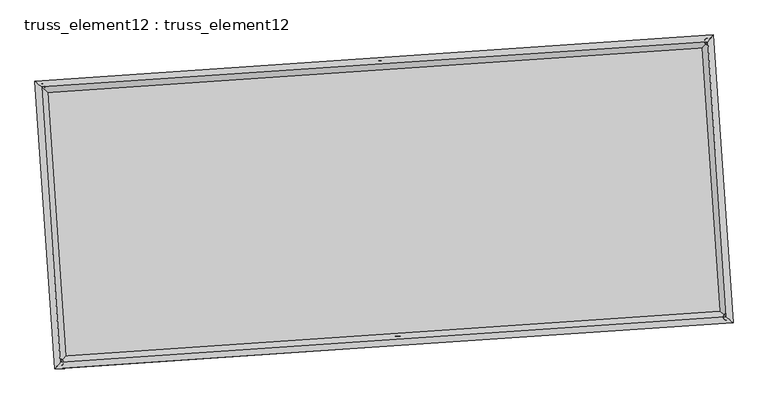
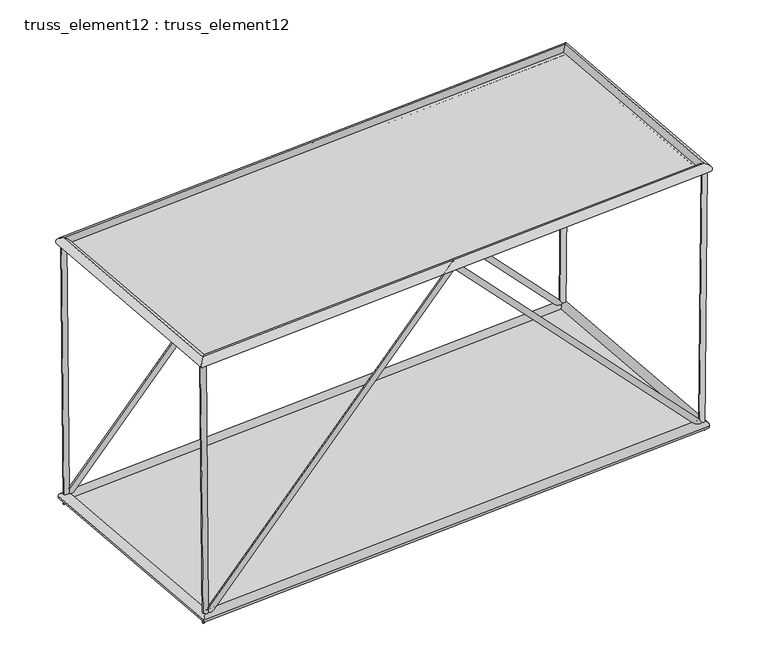
"""IFC4 building model written with IfcOpenShell, lengths in millimetres: plate geometry, truss_element12 : truss_element12."""

import ifcopenshell
import ifcopenshell.guid

model = None  # the IFC model being written
_history = None  # IfcOwnerHistory: only IFC2X3 demands one
_inside = {}  # id of a spatial element -> (the spatial element, [elements in it])
_under = {}  # id of a project, library or spatial element -> (it, [spatial elements below it])
_declared = {}  # id of a project -> (the project, [libraries it declares])
_typed = {}  # id of a type object -> (the type object, [elements of that type])
_made_of = {}  # id of a material, layer set ... -> (it, [elements and type objects made of it])


def new_model(schema):
    """Start an empty IFC model of exactly this schema.

    Asked for "IFC4X3", IfcOpenShell would pick the latest addendum, in which some entities
    have other attributes; the version numbers below select the first issue.
    IFC2X3 requires an IfcOwnerHistory on every rooted entity: one is made here for all.
    """
    global model, _history
    if schema == "IFC4X3":
        model = ifcopenshell.file(schema_version=(4, 3, 0, 0))
    else:
        model = ifcopenshell.file(schema=schema)
    _inside.clear()
    _under.clear()
    _declared.clear()
    _typed.clear()
    _made_of.clear()
    _history = None
    if model.schema == "IFC2X3":
        org = make("IfcOrganization", Name="unknown")
        user = make(
            "IfcPersonAndOrganization",
            ThePerson=make("IfcPerson", FamilyName="unknown"),
            TheOrganization=org,
        )
        app = make(
            "IfcApplication",
            ApplicationDeveloper=org,
            Version="unknown",
            ApplicationFullName="unknown",
            ApplicationIdentifier="unknown",
        )
        _history = make(
            "IfcOwnerHistory",
            OwningUser=user,
            OwningApplication=app,
            ChangeAction="ADDED",
            CreationDate=0,
        )
    return model


def make(cls, **values):
    """One entity of the class cls with the attributes given. An attribute that is None is left unset."""
    return model.create_entity(
        cls, **{name: value for name, value in values.items() if value is not None}
    )


def rooted(cls, **values):
    """An entity with a GlobalId (a new one), such as an element, a storey or a relation."""
    return make(cls, GlobalId=ifcopenshell.guid.new(), OwnerHistory=_history, **values)


def si_unit(unit_type, name, prefix=None):
    """IfcSIUnit, for example si_unit("LENGTHUNIT", "METRE", prefix="MILLI")."""
    return make("IfcSIUnit", UnitType=unit_type, Prefix=prefix, Name=name)


def assignment(units):
    """IfcUnitAssignment: the units of a project."""
    return None if units is None else make("IfcUnitAssignment", Units=units)


def point(xyz):
    """IfcCartesianPoint."""
    return None if xyz is None else make("IfcCartesianPoint", Coordinates=xyz)


def direction(xyz):
    """IfcDirection."""
    return None if xyz is None else make("IfcDirection", DirectionRatios=xyz)


def frame(location, z_axis=None, x_axis=None):
    """IfcAxis2Placement3D, a coordinate frame: its origin and axes. An axis left out is left unset."""
    return make(
        "IfcAxis2Placement3D",
        Location=point(location),
        Axis=direction(z_axis),
        RefDirection=direction(x_axis),
    )


def origin():
    """The frame at (0, 0, 0) with its axes left unset."""
    return frame((0.0, 0.0, 0.0))


def origin_with_axes():
    """The frame at (0, 0, 0) with the z axis (0, 0, 1) and the x axis (1, 0, 0) written out."""
    return frame((0.0, 0.0, 0.0), z_axis=(0.0, 0.0, 1.0), x_axis=(1.0, 0.0, 0.0))


def place(relative_to, where):
    """IfcLocalPlacement: puts the frame where relative to a parent placement (None: the world)."""
    return make(
        "IfcLocalPlacement", PlacementRelTo=relative_to, RelativePlacement=where
    )


def context(
    kind, dimensions, precision=None, world=None, true_north=None, identifier=None
):
    """IfcGeometricRepresentationContext, for example the 3D "Model" context."""
    return make(
        "IfcGeometricRepresentationContext",
        ContextIdentifier=identifier,
        ContextType=kind,
        CoordinateSpaceDimension=dimensions,
        Precision=precision,
        WorldCoordinateSystem=world,
        TrueNorth=true_north,
    )


def project(units=None, contexts=None):
    """IfcProject with its units and contexts."""
    return rooted(
        "IfcProject",
        Name="project",
        RepresentationContexts=contexts,
        UnitsInContext=assignment(units),
    )


def spatial(cls, under=None, at=None, **own):
    """A site, building, storey or space (cls), placed at a placement, below another one or the project."""
    s = rooted(cls, ObjectPlacement=at, **own)
    if under is not None:
        _under.setdefault(under.id(), (under, []))[1].append(s)
    return s


def polyline(points):
    """IfcPolyline through the points."""
    return make("IfcPolyline", Points=[point(p) for p in points])


def circle_curve(where, radius):
    """IfcCircle in the frame where."""
    return make("IfcCircle", Position=where, Radius=radius)


def ellipse_curve(where, semi_axis1, semi_axis2):
    """IfcEllipse in the frame where."""
    return make(
        "IfcEllipse", Position=where, SemiAxis1=semi_axis1, SemiAxis2=semi_axis2
    )


def outline(outer, holes=None, kind="AREA"):
    """IfcArbitraryClosedProfileDef: a profile drawn as a closed curve; with holes, ...WithVoids."""
    if holes is None:
        return make("IfcArbitraryClosedProfileDef", ProfileType=kind, OuterCurve=outer)
    return make(
        "IfcArbitraryProfileDefWithVoids",
        ProfileType=kind,
        OuterCurve=outer,
        InnerCurves=holes,
    )


def extrude(swept, where, along, depth):
    """IfcExtrudedAreaSolid: the profile swept, set in the frame where, extruded along a direction by depth."""
    return make(
        "IfcExtrudedAreaSolid",
        SweptArea=swept,
        Position=where,
        ExtrudedDirection=direction(along),
        Depth=depth,
    )


def shape(context_of_items, identifier, shape_type, items):
    """IfcShapeRepresentation: the items that make up one representation, for example the "Body"."""
    return make(
        "IfcShapeRepresentation",
        ContextOfItems=context_of_items,
        RepresentationIdentifier=identifier,
        RepresentationType=shape_type,
        Items=items,
    )


def source(mapping_origin, context_of_items, identifier, shape_type, items):
    """IfcRepresentationMap: a shape defined once, which mapped items show again and again."""
    return make(
        "IfcRepresentationMap",
        MappingOrigin=mapping_origin,
        MappedRepresentation=shape(context_of_items, identifier, shape_type, items),
    )


def transform(
    local_origin,
    x_axis=None,
    y_axis=None,
    z_axis=None,
    scale=None,
    scale2=None,
    scale3=None,
    uniform=True,
):
    """IfcCartesianTransformationOperator3D, or its non-uniform kind. x_axis, y_axis, z_axis: its Axis1, 2, 3."""
    if uniform:
        return make(
            "IfcCartesianTransformationOperator3D",
            Axis1=direction(x_axis),
            Axis2=direction(y_axis),
            LocalOrigin=point(local_origin),
            Scale=scale,
            Axis3=direction(z_axis),
        )
    return make(
        "IfcCartesianTransformationOperator3DnonUniform",
        Axis1=direction(x_axis),
        Axis2=direction(y_axis),
        LocalOrigin=point(local_origin),
        Scale=scale,
        Axis3=direction(z_axis),
        Scale2=scale2,
        Scale3=scale3,
    )


def mapped(mapping_source, mapping_target):
    """IfcMappedItem: shows the shape of a source again, moved by a transform."""
    return make(
        "IfcMappedItem", MappingSource=mapping_source, MappingTarget=mapping_target
    )


def made_of(thing, what):
    """Note that an element or type object is made of a material, layer set ...; save() writes the relation."""
    if what is not None:
        _made_of.setdefault(what.id(), (what, []))[1].append(thing)
    return thing


def element(
    cls,
    number,
    at=None,
    inside=None,
    cuts=None,
    type_object=None,
    material=None,
    context=None,
    identifier="Body",
    shape_type=None,
    held_by="IfcProductDefinitionShape",
    body=None,
    shapes=None,
    **own,
):
    """One element of the class cls, such as IfcWall. Its Tag is "e" and its number.

    at: its placement. inside: the storey or other place that contains it. cuts: it is an
    opening in that element (IfcRelVoidsElement). A single representation is given by context,
    identifier, shape_type and body (its items); several are given by shapes. held_by: the class
    of the entity that holds the representations. save() writes the other relations.
    """
    e = rooted(cls, Tag="e%d" % number, ObjectPlacement=at, **own)
    if body is not None:
        shapes = [shape(context, identifier, shape_type, body)]
    if shapes is not None:
        e.Representation = make(held_by, Representations=shapes)
    if inside is not None:
        _inside.setdefault(inside.id(), (inside, []))[1].append(e)
    if cuts is not None:
        rooted(
            "IfcRelVoidsElement", RelatingBuildingElement=cuts, RelatedOpeningElement=e
        )
    if type_object is not None:
        _typed.setdefault(type_object.id(), (type_object, []))[1].append(e)
    return made_of(e, material)


def aggregate(whole, parts):
    """IfcRelAggregates: a whole, such as a stair, and the parts it consists of."""
    return rooted("IfcRelAggregates", RelatingObject=whole, RelatedObjects=parts)


def save(model, path):
    """Write the relations noted so far, then the file.

    IfcRelAggregates (storeys below a building ...), IfcRelContainedInSpatialStructure (elements
    in a storey), IfcRelDefinesByType, IfcRelAssociatesMaterial and IfcRelDeclares: one each for
    every whole, place, type object, material and project.
    """
    for whole, parts in _under.values():
        aggregate(whole, parts)
    for where, things in _inside.values():
        rooted(
            "IfcRelContainedInSpatialStructure",
            RelatedElements=things,
            RelatingStructure=where,
        )
    for kind, things in _typed.values():
        rooted("IfcRelDefinesByType", RelatedObjects=things, RelatingType=kind)
    for what, things in _made_of.values():
        rooted("IfcRelAssociatesMaterial", RelatedObjects=things, RelatingMaterial=what)
    for by, libraries in _declared.values():
        rooted("IfcRelDeclares", RelatingContext=by, RelatedDefinitions=libraries)
    model.write(path)


def plane_surface(at):
    """IfcPlane: the flat surface through the origin of the frame at, square to its z axis."""
    return make("IfcPlane", Position=at)


def cylinder_surface(at, radius):
    """IfcCylindricalSurface: all points at the distance radius from the z axis of the frame at."""
    return make("IfcCylindricalSurface", Position=at, Radius=radius)


def advanced_brep(points, edges, surfaces, faces):
    """IfcAdvancedBrep: a solid bounded by faces that lie on surfaces and meet in shared edges.

    An edge is (start, end): straight between two places in points (the first is 0);
    or (start, end, curve); or (start, end, curve, False) where it runs against its curve.
    A face is (place in surfaces, loops), or (place, loops, False) where it looks against
    its surface's normal. A loop lists edges by number (the first is 1), with a minus sign
    where the edge is run from its end to its start. The first loop is the outer one.
    """
    corners = [point(p) for p in points]
    vertices = [make("IfcVertexPoint", VertexGeometry=c) for c in corners]
    made = []
    for start, end, *more in edges:
        made.append(
            make(
                "IfcEdgeCurve",
                EdgeStart=vertices[start],
                EdgeEnd=vertices[end],
                EdgeGeometry=more[0] if more else make("IfcPolyline", Points=[corners[start], corners[end]]),
                SameSense=more[1] if len(more) > 1 else True,
            )
        )
    hull = []
    for where, loops, *sense in faces:
        bounds = []
        for j, loop in enumerate(loops):
            ring = [make("IfcOrientedEdge", EdgeElement=made[abs(k) - 1], Orientation=k > 0) for k in loop]
            bounds.append(
                make(
                    "IfcFaceOuterBound" if j == 0 else "IfcFaceBound",
                    Bound=make("IfcEdgeLoop", EdgeList=ring),
                    Orientation=True,
                )
            )
        hull.append(make("IfcAdvancedFace", Bounds=bounds, FaceSurface=surfaces[where], SameSense=sense[0] if sense else True))
    return make("IfcAdvancedBrep", Outer=make("IfcClosedShell", CfsFaces=hull))


def truss_element12_truss_element12_3d995396(model_context):
    return source(origin(), model_context, "Body", "SolidModel", [
        advanced_brep(
        [(-3712.6408018, 2272.9715483, 5000.2484753), (-3811.7396164, 2259.6106092, 4999.2944024), (-3666.1125982, 2276.1441296, 122.9707334), (-3762.8742846, 2262.9425505, -122.9707334), (1064.1401196, 2598.6820811, 5071.8896086), (1064.5820396, 2592.1084463, 4927.6451952), (5793.5718475, 2921.1640524, 122.9648431), (5891.1891295, 2921.2164361, -122.9648431), (5840.9148394, 2924.392191, 5000.2487538), (5940.9098971, 2924.6067063, 4999.2779762)],
        [
            (0, 1, circle_curve(frame((-3762.1902091, 2266.2910788, 4999.7714389), z_axis=(-0.009539353531426898, -0.0006504522548332356, 0.9999542877782298), x_axis=(-0.13360948886072543, 0.9910338579689815, -0.0006299567385858392)), 50.0)),
            (1, 0, circle_curve(frame((-3762.1902091, 2266.2910788, 4999.7714389), z_axis=(-0.009539353531426898, -0.0006504522548332356, 0.9999542877782298), x_axis=(-0.13360948886072543, 0.9910338579689815, -0.0006299567385858392)), 50.0)),
            (0, 2),
            (2, 3, ellipse_curve(frame((-3714.4934414, 2269.54334, 0.0), z_axis=(-0.9275444537546121, -0.06324573037496291, 0.368322228352289), x_axis=(0.3674689716323781, 0.02505631229527238, 0.9296981962452139)), 132.5575344, 50.0)),
            (3, 1),
            (3, 2, ellipse_curve(frame((-3714.4934414, 2269.54334, 0.0), z_axis=(-0.9275444537546121, -0.06324573037496291, 0.368322228352289), x_axis=(0.3674689716323781, 0.02505631229527238, 0.9296981962452139)), 132.5575344, 50.0)),
            (2, 4),
            (4, 5, ellipse_curve(frame((1064.3610796, 2595.3952637, 4999.7674019), z_axis=(-0.9976833951243609, -0.06802823816388774, 4.365141464773057e-05), x_axis=(-4.355029160929896e-05, -2.969528831717673e-06, -0.9999999990472769)), 72.279252, 50.0)),
            (5, 3),
            (5, 4, ellipse_curve(frame((1064.3610796, 2595.3952637, 4999.7674019), z_axis=(-0.9976833951243609, -0.06802823816388774, 4.365141464773057e-05), x_axis=(-4.355029160929896e-05, -2.969528831717673e-06, -0.9999999990472769)), 72.279252, 50.0)),
            (4, 6),
            (6, 7, ellipse_curve(frame((5842.3804885, 2921.1902443, 0.0), z_axis=(-0.9275912472386779, -0.06324892104476065, -0.36820381860169205), x_axis=(-0.36735083619027376, -0.02504825708855556, 0.9297450983829559)), 132.5444982, 50.0)),
            (7, 5),
            (7, 6, ellipse_curve(frame((5842.3804885, 2921.1902443, 0.0), z_axis=(-0.9275912472386779, -0.06324892104476065, -0.36820381860169205), x_axis=(-0.36735083619027376, -0.02504825708855556, 0.9297450983829559)), 132.5444982, 50.0)),
            (8, 9, circle_curve(frame((5890.9123683, 2924.4994486, 4999.763365), z_axis=(0.009706375954598431, 0.0006618408789518583, 0.999952672996317), x_axis=(-0.0021514761027001668, 0.999997480140261, -0.0006409865112665113)), 50.0)),
            (9, 8, circle_curve(frame((5890.9123683, 2924.4994486, 4999.763365), z_axis=(0.009706375954598431, 0.0006618408789518583, 0.999952672996317), x_axis=(-0.0021514761027001668, 0.999997480140261, -0.0006409865112665113)), 50.0)),
            (6, 8),
            (9, 7),
        ],
        [
            plane_surface(frame((-3762.1902091, 2316.2910682, 4999.803963), z_axis=(-0.009539353531428214, -0.0006504522548355754, 0.9999542877782297), x_axis=(0.9999544993319458, -6.205176354079358e-06, 0.009539351513250697))),
            cylinder_surface(frame((-3762.1902091, 2266.2910788, 4999.7714389), z_axis=(-0.009539353531426898, -0.0006504522548332356, 0.9999542877782298), x_axis=(-0.13360948886072543, 0.9910338579689815, -0.0006299567385858392)), 50.0),
            cylinder_surface(frame((-3714.4934414, 2269.54334, 0.0), z_axis=(-0.6901903584114236, -0.0470614568808942, -0.7220958997475049), x_axis=(-0.020415575362847597, 0.998752120640053, -0.04557856732721049)), 50.0),
            cylinder_surface(frame((1064.3610796, 2595.3952637, 4999.7674019), z_axis=(-0.6901274608072349, -0.047057168132365004, 0.7221562924790736), x_axis=(-0.11534925319653908, 0.9922789540252682, -0.04557441371559841)), 50.0),
            plane_surface(frame((5890.9123683, 2874.4994596, 4999.7964586), z_axis=(0.009706375954601498, 0.0006618408789477092, 0.9999526729963171), x_axis=(0.9999528920233334, -6.42437903231041e-06, -0.009706373828542777))),
            cylinder_surface(frame((5842.3804885, 2921.1902443, 0.0), z_axis=(-0.00970637595459843, -0.0006618408789518581, -0.9999526729963167), x_axis=(-0.0021514761027001668, 0.999997480140261, -0.0006409865112665113)), 50.0),
        ],
        [
            (0, [[1, 2]]),
            (1, [[-1, 3, 4, 5]]),
            (1, [[-2, -5, 6, -3]]),
            (2, [[-4, 7, 8, 9]]),
            (2, [[-6, -9, 10, -7]]),
            (3, [[-8, 11, 12, 13]]),
            (3, [[-10, -13, 14, -11]]),
            (4, [[15, 16]]),
            (5, [[-12, 17, -16, 18]]),
            (5, [[-14, -18, -15, -17]]),
        ],
    ),
        advanced_brep(
        [(-3440.5278489, -1717.762036, 5000.2484753), (-3539.6266635, -1731.1229751, 4999.2944024), (-3393.9996453, -1714.5894547, 122.9707334), (-3490.7613317, -1727.7910338, -122.9707334), (1336.2530725, -1392.0515032, 5071.8896086), (1336.6949926, -1398.625138, 4927.6451952), (6065.6848004, -1069.5695319, 122.9648431), (6163.3020824, -1069.5171482, -122.9648431), (6113.0277923, -1066.3413933, 5000.2487538), (6213.0228501, -1066.126878, 4999.2779762)],
        [
            (0, 1, circle_curve(frame((-3490.0772562, -1724.4425055, 4999.7714389), z_axis=(-0.009539353531426684, -0.0006504522548331923, 0.9999542877782298), x_axis=(-0.1336094888607254, 0.9910338579689815, -0.0006299567385858533)), 50.0)),
            (1, 0, circle_curve(frame((-3490.0772562, -1724.4425055, 4999.7714389), z_axis=(-0.009539353531426684, -0.0006504522548331923, 0.9999542877782298), x_axis=(-0.1336094888607254, 0.9910338579689815, -0.0006299567385858533)), 50.0)),
            (0, 2),
            (2, 3, ellipse_curve(frame((-3442.3804885, -1721.1902443, 0.0), z_axis=(-0.9275444537546114, -0.06324573037496278, 0.3683222283522907), x_axis=(0.36746897163237974, 0.025056312295272495, 0.9296981962452131)), 132.5575344, 50.0)),
            (3, 1),
            (3, 2, ellipse_curve(frame((-3442.3804885, -1721.1902443, 0.0), z_axis=(-0.9275444537546114, -0.06324573037496278, 0.3683222283522907), x_axis=(0.36746897163237974, 0.025056312295272495, 0.9296981962452131)), 132.5575344, 50.0)),
            (2, 4),
            (4, 5, ellipse_curve(frame((1336.4740325, -1395.3383206, 4999.7674019), z_axis=(-0.9976833951243609, -0.06802823816388762, 4.365141464997738e-05), x_axis=(-4.355029161160519e-05, -2.9695288319579026e-06, -0.9999999990472771)), 72.279252, 50.0)),
            (5, 3),
            (5, 4, ellipse_curve(frame((1336.4740325, -1395.3383206, 4999.7674019), z_axis=(-0.9976833951243609, -0.06802823816388762, 4.365141464997738e-05), x_axis=(-4.355029161160519e-05, -2.9695288319579026e-06, -0.9999999990472771)), 72.279252, 50.0)),
            (4, 6),
            (6, 7, ellipse_curve(frame((6114.4934414, -1069.54334, 0.0), z_axis=(-0.927591247238678, -0.06324892104476053, -0.3682038186016914), x_axis=(-0.3673508361902732, -0.025048257088555438, 0.929745098382956)), 132.5444982, 50.0)),
            (7, 5),
            (7, 6, ellipse_curve(frame((6114.4934414, -1069.54334, 0.0), z_axis=(-0.927591247238678, -0.06324892104476053, -0.3682038186016914), x_axis=(-0.3673508361902732, -0.025048257088555438, 0.929745098382956)), 132.5444982, 50.0)),
            (8, 9, circle_curve(frame((6163.0253212, -1066.2341357, 4999.763365), z_axis=(0.009706375954599215, 0.0006618408789519453, 0.999952672996317), x_axis=(-0.002151476102700382, 0.9999974801402611, -0.0006409865112665946)), 50.0)),
            (9, 8, circle_curve(frame((6163.0253212, -1066.2341357, 4999.763365), z_axis=(0.009706375954599215, 0.0006618408789519453, 0.999952672996317), x_axis=(-0.002151476102700382, 0.9999974801402611, -0.0006409865112665946)), 50.0)),
            (6, 8),
            (9, 7),
        ],
        [
            plane_surface(frame((-3490.0772562, -1674.4425161, 4999.803963), z_axis=(-0.009539353531428214, -0.0006504522548355842, 0.9999542877782297), x_axis=(0.9999544993319458, -6.205176354079358e-06, 0.009539351513250697))),
            cylinder_surface(frame((-3490.0772562, -1724.4425055, 4999.7714389), z_axis=(-0.009539353531426684, -0.0006504522548331923, 0.9999542877782298), x_axis=(-0.1336094888607254, 0.9910338579689815, -0.0006299567385858533)), 50.0),
            cylinder_surface(frame((-3442.3804885, -1721.1902443, 0.0), z_axis=(-0.6901903584114265, -0.047061456880894366, -0.7220958997475021), x_axis=(-0.020415575362847802, 0.998752120640053, -0.04557856732721061)), 50.0),
            cylinder_surface(frame((1336.4740325, -1395.3383206, 4999.7674019), z_axis=(-0.6901274608072342, -0.047057168132364824, 0.722156292479074), x_axis=(-0.1153492531965389, 0.9922789540252682, -0.04557441371559837)), 50.0),
            plane_surface(frame((6163.0253212, -1116.2341247, 4999.7964586), z_axis=(0.009706375954601498, 0.0006618408789477163, 0.9999526729963171), x_axis=(0.9999528920233334, -6.424379032754499e-06, -0.009706373828542777))),
            cylinder_surface(frame((6114.4934414, -1069.54334, 0.0), z_axis=(-0.009706375954599215, -0.0006618408789519453, -0.999952672996317), x_axis=(-0.002151476102700382, 0.9999974801402611, -0.0006409865112665946)), 50.0),
        ],
        [
            (0, [[1, 2]]),
            (1, [[-1, 3, 4, 5]]),
            (1, [[-2, -5, 6, -3]]),
            (2, [[-4, 7, 8, 9]]),
            (2, [[-6, -9, 10, -7]]),
            (3, [[-8, 11, 12, 13]]),
            (3, [[-10, -13, 14, -11]]),
            (4, [[15, 16]]),
            (5, [[-12, 17, -16, 18]]),
            (5, [[-14, -18, -15, -17]]),
        ],
    ),
        advanced_brep(
        [(-3490.0793814, -1724.444861, 4909.7714389), (-3490.075131, -1724.4401501, 5089.7714389), (-3762.1877838, 2266.2890336, 5089.7714389), (-3762.1926343, 2266.2931239, 4909.7714389), (5890.9103929, 2924.4971034, 5089.763365), (5890.9143436, 2924.5017939, 4909.763365), (6163.0230458, -1066.2320803, 5089.763365), (6163.0275966, -1066.236191, 4909.763365)],
        [
            (0, 1, ellipse_curve(frame((-3490.0772562, -1724.4425055, 4999.7714389), z_axis=(-0.7535719234052061, 0.6573654662781049, 5.900579994198024e-07), x_axis=(-0.6573654662778425, -0.7535719234054348, 5.900580116710992e-07)), 127.2792206, 90.0)),
            (1, 2),
            (2, 3, ellipse_curve(frame((-3762.1902091, 2266.2910788, 4999.7714389), z_axis=(-0.6573654662778421, -0.7535719234054352, 5.900580091387355e-07), x_axis=(0.7535719234052064, -0.6573654662781044, -5.900579968874395e-07)), 127.2792206, 90.0)),
            (3, 0),
            (1, 0, ellipse_curve(frame((-3490.0772562, -1724.4425055, 4999.7714389), z_axis=(-0.7535719234052061, 0.6573654662781049, 5.900579994198024e-07), x_axis=(-0.6573654662778425, -0.7535719234054348, 5.900580116710992e-07)), 127.2792206, 90.0)),
            (3, 2, ellipse_curve(frame((-3762.1902091, 2266.2910788, 4999.7714389), z_axis=(-0.6573654662778421, -0.7535719234054352, 5.900580091387355e-07), x_axis=(0.7535719234052064, -0.6573654662781044, -5.900579968874395e-07)), 127.2792206, 90.0)),
            (2, 4),
            (4, 5, ellipse_curve(frame((5890.9123683, 2924.4994486, 4999.763365), z_axis=(-0.753571923405209, 0.6573654662781013, 5.90058003013114e-07), x_axis=(-0.6573654662778391, -0.7535719234054377, 5.900580030130607e-07)), 127.2792206, 90.0)),
            (5, 3),
            (5, 4, ellipse_curve(frame((5890.9123683, 2924.4994486, 4999.763365), z_axis=(-0.753571923405209, 0.6573654662781013, 5.90058003013114e-07), x_axis=(-0.6573654662778391, -0.7535719234054377, 5.900580030130607e-07)), 127.2792206, 90.0)),
            (4, 6),
            (6, 7, ellipse_curve(frame((6163.0253212, -1066.2341357, 4999.763365), z_axis=(0.6573654662778391, 0.7535719234054377, -5.900580055454242e-07), x_axis=(-0.7535719234052087, 0.6573654662781017, 5.900580055454772e-07)), 127.2792206, 90.0)),
            (7, 5),
            (7, 6, ellipse_curve(frame((6163.0253212, -1066.2341357, 4999.763365), z_axis=(0.6573654662778391, 0.7535719234054377, -5.900580055454242e-07), x_axis=(-0.7535719234052087, 0.6573654662781017, 5.900580055454772e-07)), 127.2792206, 90.0)),
            (6, 1),
            (0, 7),
        ],
        [
            cylinder_surface(frame((-3490.0772562, -1724.4425055, 4999.7714389), z_axis=(0.06802823822868706, -0.9976833960748777, 0.0), x_axis=(-0.9976833957545878, -0.06802823820684771, 2.53390411256576e-05)), 90.0),
            cylinder_surface(frame((-3762.1902091, 2266.2910788, 4999.7714389), z_axis=(-0.9976833960745297, -0.06802823822867328, 8.344680304478929e-07), x_axis=(-0.06802823818787146, 0.9976833957767265, 2.450457308679736e-05)), 90.0),
            cylinder_surface(frame((5890.9123683, 2924.4994486, 4999.763365), z_axis=(-0.06802823822869537, 0.9976833960748771, 0.0), x_axis=(0.9976833957953891, 0.06802823820963814, 2.3670105056600042e-05)), 90.0),
            cylinder_surface(frame((6163.0253212, -1066.2341357, 4999.763365), z_axis=(0.9976833960745297, 0.06802823822867272, -8.344680340291955e-07), x_axis=(0.06802823822867272, -0.9976833957739445, 2.450457309037874e-05)), 90.0),
        ],
        [
            (0, [[1, 2, 3, 4]]),
            (0, [[5, -4, 6, -2]]),
            (1, [[-3, 7, 8, 9]]),
            (1, [[-6, -9, 10, -7]]),
            (2, [[-8, 11, 12, 13]]),
            (2, [[-10, -13, 14, -11]]),
            (3, [[-12, 15, -1, 16]]),
            (3, [[-14, -16, -5, -15]]),
        ],
    ),
        advanced_brep(
        [(-3358.7115243, -1625.2761972, 0.0), (-3526.0494527, -1817.1042913, 0.0), (-3810.4074885, 2353.2123043, 0.0), (-3618.5793943, 2185.8743758, 0.0), (5926.0494527, 3017.1042913, 0.0), (5758.7115243, 2825.2761972, 0.0), (6210.4074885, -1153.2123043, 0.0), (6018.5793943, -985.8743758, 0.0)],
        [
            (0, 1, ellipse_curve(frame((-3442.3804885, -1721.1902443, 0.0), z_axis=(-0.7535719234054536, 0.6573654662780856, 0.0), x_axis=(-0.6573654662780855, -0.7535719234054539, 0.0)), 127.2792206, 90.0)),
            (1, 2),
            (2, 3, ellipse_curve(frame((-3714.4934414, 2269.54334, 0.0), z_axis=(-0.6573654662780855, -0.7535719234054539, 0.0), x_axis=(0.7535719234054538, -0.6573654662780856, 0.0)), 127.2792206, 90.0)),
            (3, 0),
            (1, 0, ellipse_curve(frame((-3442.3804885, -1721.1902443, 0.0), z_axis=(-0.7535719234054536, 0.6573654662780856, 0.0), x_axis=(-0.6573654662780855, -0.7535719234054539, 0.0)), 127.2792206, 90.0)),
            (3, 2, ellipse_curve(frame((-3714.4934414, 2269.54334, 0.0), z_axis=(-0.6573654662780855, -0.7535719234054539, 0.0), x_axis=(0.7535719234054538, -0.6573654662780856, 0.0)), 127.2792206, 90.0)),
            (2, 4),
            (4, 5, ellipse_curve(frame((5842.3804885, 2921.1902443, 0.0), z_axis=(-0.7535719234054568, 0.6573654662780822, 0.0), x_axis=(-0.657365466278082, -0.7535719234054568, 0.0)), 127.2792206, 90.0)),
            (5, 3),
            (5, 4, ellipse_curve(frame((5842.3804885, 2921.1902443, 0.0), z_axis=(-0.7535719234054568, 0.6573654662780822, 0.0), x_axis=(-0.657365466278082, -0.7535719234054568, 0.0)), 127.2792206, 90.0)),
            (4, 6),
            (6, 7, ellipse_curve(frame((6114.4934414, -1069.54334, 0.0), z_axis=(0.6573654662780823, 0.7535719234054566, 0.0), x_axis=(-0.7535719234054565, 0.6573654662780822, 0.0)), 127.2792206, 90.0)),
            (7, 5),
            (7, 6, ellipse_curve(frame((6114.4934414, -1069.54334, 0.0), z_axis=(0.6573654662780823, 0.7535719234054566, 0.0), x_axis=(-0.7535719234054565, 0.6573654662780822, 0.0)), 127.2792206, 90.0)),
            (6, 1),
            (0, 7),
        ],
        [
            cylinder_surface(frame((-3442.3804885, -1721.1902443, 0.0), z_axis=(0.06802823822869013, -0.9976833960748773, 0.0), x_axis=(-0.9976833960748773, -0.06802823822869013, 0.0)), 90.0),
            cylinder_surface(frame((-3714.4934414, 2269.54334, 0.0), z_axis=(-0.9976833960748767, -0.06802823822869991, 0.0), x_axis=(-0.06802823822869991, 0.9976833960748767, 0.0)), 90.0),
            cylinder_surface(frame((5842.3804885, 2921.1902443, 0.0), z_axis=(-0.06802823822869869, 0.9976833960748768, 0.0), x_axis=(0.9976833960748768, 0.06802823822869869, 0.0)), 90.0),
            cylinder_surface(frame((6114.4934414, -1069.54334, 0.0), z_axis=(0.9976833960748768, 0.06802823822869974, 0.0), x_axis=(0.06802823822869974, -0.9976833960748768, 0.0)), 90.0),
        ],
        [
            (0, [[1, 2, 3, 4]]),
            (0, [[5, -4, 6, -2]]),
            (1, [[-3, 7, 8, 9]]),
            (1, [[-6, -9, 10, -7]]),
            (2, [[-8, 11, 12, 13]]),
            (2, [[-10, -13, 14, -11]]),
            (3, [[-12, 15, -1, 16]]),
            (3, [[-14, -16, -5, -15]]),
        ],
    ),
        extrude(outline(polyline([(-3442.3804885, -1721.1902443), (-3714.4934414, 2269.54334), (5842.3804885, 2921.1902443), (6114.4934414, -1069.54334), (-3442.3804885, -1721.1902443)])), origin_with_axes(), (0.0, 0.0, 1.0), 20.0),
        extrude(outline(polyline([(-2000.0, 4837.758459), (2000.0, 4837.758459), (1999.9999999, -4837.7584589), (-2000.0000001, -4837.7584589), (-2000.0, 4837.758459)])), frame((1200.4175561, 600.0284716, 4999.7674019), z_axis=(8.32534897943804e-07, 5.67673986124007e-08, 0.999999999999652), x_axis=(-0.06802823822868996, 0.9976833960748774, 0.0)), (0.0, 0.0, 1.0), 20.0),
    ])


if __name__ == "__main__":
    model = new_model("IFC4")
    model_context = context("Model", 3, world=origin())
    ifc_project = project(units=[si_unit("LENGTHUNIT", "METRE", prefix="MILLI")], contexts=[model_context])
    site = spatial("IfcSite", under=ifc_project)
    building = spatial("IfcBuilding", under=site)
    placement = place(None, origin())
    truss_element12_truss_element12_shape = truss_element12_truss_element12_3d995396(model_context)
    element("IfcPlate", 1, ObjectType="truss_element12 : truss_element12", at=placement, inside=building, context=model_context, shape_type="MappedRepresentation", body=[
        mapped(truss_element12_truss_element12_shape, transform((0.0, 0.0, 0.0), x_axis=(1.0, 0.0, 0.0), y_axis=(0.0, 1.0, 0.0), z_axis=(0.0, 0.0, 1.0))),
    ])
    save(model, "model.ifc")

# Revit data of these elements
# Type "truss_element12 : truss_element12"
#   steellbar1 = 90 mm
#   steelbar2 = 50 mm
#   offset1 = 5000 mm
#   M = Default Roof
# Element 1 (IfcPlate, "truss_element12 : truss_element12")
#   Materials on its faces: "Default Roof"
# Materials
#   "Default Roof": class "Miscellaneous", colour RGB 0 127 0, transparency 0, Comments = "Rendering appearance not upgraded Rendering appearance not upgraded ", Cost = 0
